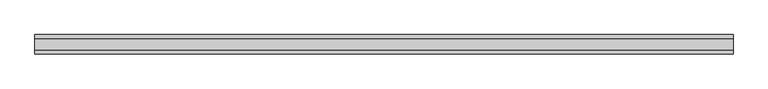
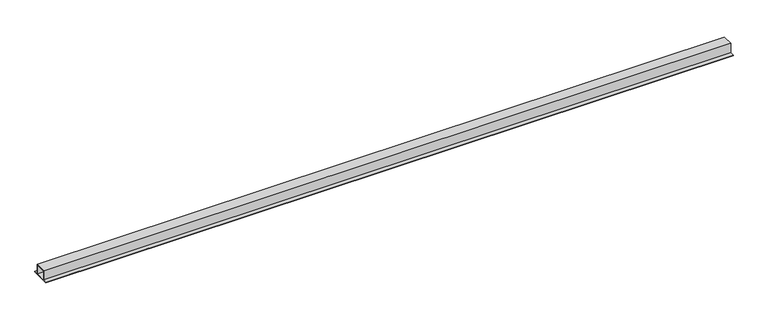
"""IFC4 building model written with IfcOpenShell, lengths in millimetres: beam geometry, NLRS_28_SF_LIB_stalen ligger THQ-AV-CWV-MMBS-SRP_gen_rsf : stalen ligger_gen__THQ_280x10-290x30-550x20."""

import ifcopenshell
import ifcopenshell.guid

model = None  # the IFC model being written
_history = None  # IfcOwnerHistory: only IFC2X3 demands one
_inside = {}  # id of a spatial element -> (the spatial element, [elements in it])
_under = {}  # id of a project, library or spatial element -> (it, [spatial elements below it])
_declared = {}  # id of a project -> (the project, [libraries it declares])
_typed = {}  # id of a type object -> (the type object, [elements of that type])
_made_of = {}  # id of a material, layer set ... -> (it, [elements and type objects made of it])


def new_model(schema):
    """Start an empty IFC model of exactly this schema.

    Asked for "IFC4X3", IfcOpenShell would pick the latest addendum, in which some entities
    have other attributes; the version numbers below select the first issue.
    IFC2X3 requires an IfcOwnerHistory on every rooted entity: one is made here for all.
    """
    global model, _history
    if schema == "IFC4X3":
        model = ifcopenshell.file(schema_version=(4, 3, 0, 0))
    else:
        model = ifcopenshell.file(schema=schema)
    _inside.clear()
    _under.clear()
    _declared.clear()
    _typed.clear()
    _made_of.clear()
    _history = None
    if model.schema == "IFC2X3":
        org = make("IfcOrganization", Name="unknown")
        user = make(
            "IfcPersonAndOrganization",
            ThePerson=make("IfcPerson", FamilyName="unknown"),
            TheOrganization=org,
        )
        app = make(
            "IfcApplication",
            ApplicationDeveloper=org,
            Version="unknown",
            ApplicationFullName="unknown",
            ApplicationIdentifier="unknown",
        )
        _history = make(
            "IfcOwnerHistory",
            OwningUser=user,
            OwningApplication=app,
            ChangeAction="ADDED",
            CreationDate=0,
        )
    return model


def make(cls, **values):
    """One entity of the class cls with the attributes given. An attribute that is None is left unset."""
    return model.create_entity(
        cls, **{name: value for name, value in values.items() if value is not None}
    )


def rooted(cls, **values):
    """An entity with a GlobalId (a new one), such as an element, a storey or a relation."""
    return make(cls, GlobalId=ifcopenshell.guid.new(), OwnerHistory=_history, **values)


def si_unit(unit_type, name, prefix=None):
    """IfcSIUnit, for example si_unit("LENGTHUNIT", "METRE", prefix="MILLI")."""
    return make("IfcSIUnit", UnitType=unit_type, Prefix=prefix, Name=name)


def assignment(units):
    """IfcUnitAssignment: the units of a project."""
    return None if units is None else make("IfcUnitAssignment", Units=units)


def point(xyz):
    """IfcCartesianPoint."""
    return None if xyz is None else make("IfcCartesianPoint", Coordinates=xyz)


def direction(xyz):
    """IfcDirection."""
    return None if xyz is None else make("IfcDirection", DirectionRatios=xyz)


def frame(location, z_axis=None, x_axis=None):
    """IfcAxis2Placement3D, a coordinate frame: its origin and axes. An axis left out is left unset."""
    return make(
        "IfcAxis2Placement3D",
        Location=point(location),
        Axis=direction(z_axis),
        RefDirection=direction(x_axis),
    )


def origin():
    """The frame at (0, 0, 0) with its axes left unset."""
    return frame((0.0, 0.0, 0.0))


def place(relative_to, where):
    """IfcLocalPlacement: puts the frame where relative to a parent placement (None: the world)."""
    return make(
        "IfcLocalPlacement", PlacementRelTo=relative_to, RelativePlacement=where
    )


def context(
    kind, dimensions, precision=None, world=None, true_north=None, identifier=None
):
    """IfcGeometricRepresentationContext, for example the 3D "Model" context."""
    return make(
        "IfcGeometricRepresentationContext",
        ContextIdentifier=identifier,
        ContextType=kind,
        CoordinateSpaceDimension=dimensions,
        Precision=precision,
        WorldCoordinateSystem=world,
        TrueNorth=true_north,
    )


def project(units=None, contexts=None):
    """IfcProject with its units and contexts."""
    return rooted(
        "IfcProject",
        Name="project",
        RepresentationContexts=contexts,
        UnitsInContext=assignment(units),
    )


def spatial(cls, under=None, at=None, **own):
    """A site, building, storey or space (cls), placed at a placement, below another one or the project."""
    s = rooted(cls, ObjectPlacement=at, **own)
    if under is not None:
        _under.setdefault(under.id(), (under, []))[1].append(s)
    return s


def polyline(points):
    """IfcPolyline through the points."""
    return make("IfcPolyline", Points=[point(p) for p in points])


def outline(outer, holes=None, kind="AREA"):
    """IfcArbitraryClosedProfileDef: a profile drawn as a closed curve; with holes, ...WithVoids."""
    if holes is None:
        return make("IfcArbitraryClosedProfileDef", ProfileType=kind, OuterCurve=outer)
    return make(
        "IfcArbitraryProfileDefWithVoids",
        ProfileType=kind,
        OuterCurve=outer,
        InnerCurves=holes,
    )


def extrude(swept, where, along, depth):
    """IfcExtrudedAreaSolid: the profile swept, set in the frame where, extruded along a direction by depth."""
    return make(
        "IfcExtrudedAreaSolid",
        SweptArea=swept,
        Position=where,
        ExtrudedDirection=direction(along),
        Depth=depth,
    )


def shape(context_of_items, identifier, shape_type, items):
    """IfcShapeRepresentation: the items that make up one representation, for example the "Body"."""
    return make(
        "IfcShapeRepresentation",
        ContextOfItems=context_of_items,
        RepresentationIdentifier=identifier,
        RepresentationType=shape_type,
        Items=items,
    )


def source(mapping_origin, context_of_items, identifier, shape_type, items):
    """IfcRepresentationMap: a shape defined once, which mapped items show again and again."""
    return make(
        "IfcRepresentationMap",
        MappingOrigin=mapping_origin,
        MappedRepresentation=shape(context_of_items, identifier, shape_type, items),
    )


def transform(
    local_origin,
    x_axis=None,
    y_axis=None,
    z_axis=None,
    scale=None,
    scale2=None,
    scale3=None,
    uniform=True,
):
    """IfcCartesianTransformationOperator3D, or its non-uniform kind. x_axis, y_axis, z_axis: its Axis1, 2, 3."""
    if uniform:
        return make(
            "IfcCartesianTransformationOperator3D",
            Axis1=direction(x_axis),
            Axis2=direction(y_axis),
            LocalOrigin=point(local_origin),
            Scale=scale,
            Axis3=direction(z_axis),
        )
    return make(
        "IfcCartesianTransformationOperator3DnonUniform",
        Axis1=direction(x_axis),
        Axis2=direction(y_axis),
        LocalOrigin=point(local_origin),
        Scale=scale,
        Axis3=direction(z_axis),
        Scale2=scale2,
        Scale3=scale3,
    )


def mapped(mapping_source, mapping_target):
    """IfcMappedItem: shows the shape of a source again, moved by a transform."""
    return make(
        "IfcMappedItem", MappingSource=mapping_source, MappingTarget=mapping_target
    )


def made_of(thing, what):
    """Note that an element or type object is made of a material, layer set ...; save() writes the relation."""
    if what is not None:
        _made_of.setdefault(what.id(), (what, []))[1].append(thing)
    return thing


def element(
    cls,
    number,
    at=None,
    inside=None,
    cuts=None,
    type_object=None,
    material=None,
    context=None,
    identifier="Body",
    shape_type=None,
    held_by="IfcProductDefinitionShape",
    body=None,
    shapes=None,
    **own,
):
    """One element of the class cls, such as IfcWall. Its Tag is "e" and its number.

    at: its placement. inside: the storey or other place that contains it. cuts: it is an
    opening in that element (IfcRelVoidsElement). A single representation is given by context,
    identifier, shape_type and body (its items); several are given by shapes. held_by: the class
    of the entity that holds the representations. save() writes the other relations.
    """
    e = rooted(cls, Tag="e%d" % number, ObjectPlacement=at, **own)
    if body is not None:
        shapes = [shape(context, identifier, shape_type, body)]
    if shapes is not None:
        e.Representation = make(held_by, Representations=shapes)
    if inside is not None:
        _inside.setdefault(inside.id(), (inside, []))[1].append(e)
    if cuts is not None:
        rooted(
            "IfcRelVoidsElement", RelatingBuildingElement=cuts, RelatedOpeningElement=e
        )
    if type_object is not None:
        _typed.setdefault(type_object.id(), (type_object, []))[1].append(e)
    return made_of(e, material)


def aggregate(whole, parts):
    """IfcRelAggregates: a whole, such as a stair, and the parts it consists of."""
    return rooted("IfcRelAggregates", RelatingObject=whole, RelatedObjects=parts)


def save(model, path):
    """Write the relations noted so far, then the file.

    IfcRelAggregates (storeys below a building ...), IfcRelContainedInSpatialStructure (elements
    in a storey), IfcRelDefinesByType, IfcRelAssociatesMaterial and IfcRelDeclares: one each for
    every whole, place, type object, material and project.
    """
    for whole, parts in _under.values():
        aggregate(whole, parts)
    for where, things in _inside.values():
        rooted(
            "IfcRelContainedInSpatialStructure",
            RelatedElements=things,
            RelatingStructure=where,
        )
    for kind, things in _typed.values():
        rooted("IfcRelDefinesByType", RelatedObjects=things, RelatingType=kind)
    for what, things in _made_of.values():
        rooted("IfcRelAssociatesMaterial", RelatedObjects=things, RelatingMaterial=what)
    for by, libraries in _declared.values():
        rooted("IfcRelDeclares", RelatingContext=by, RelatedDefinitions=libraries)
    model.write(path)


def beam_1759c74d(model_context):
    return source(origin(), model_context, "Body", "SweptSolid", [
        extrude(outline(polyline([(143.5, 280.0), (143.5, 0.0), (263.5, 0.0), (263.5, -20.0), (-286.5, -20.0), (-286.5, 0.0), (-166.5, 0.0), (-166.5, 280.0), (143.5, 280.0)]), holes=[polyline([(133.5, 0.0), (133.5, 250.0), (-156.5, 250.0), (-156.5, 0.0), (133.5, 0.0)])]), frame((-9887.5, 0.0, 0.0), z_axis=(1.0, 0.0, 0.0), x_axis=(0.0, 1.0, 0.0)), (0.0, 0.0, 1.0), 19775.0),
    ])


if __name__ == "__main__":
    model = new_model("IFC4")
    model_context = context("Model", 3, world=origin())
    ifc_project = project(units=[si_unit("LENGTHUNIT", "METRE", prefix="MILLI")], contexts=[model_context])
    site = spatial("IfcSite", under=ifc_project)
    building = spatial("IfcBuilding", under=site)
    placement = place(None, origin())
    beam_shape = beam_1759c74d(model_context)
    element("IfcBeam", 1, ObjectType="NLRS_28_SF_LIB_stalen ligger THQ-AV-CWV-MMBS-SRP_gen_rsf : stalen ligger_gen__THQ_280x10-290x30-550x20", at=placement, inside=building, context=model_context, shape_type="MappedRepresentation", body=[
        mapped(beam_shape, transform((0.0, 0.0, 0.0), x_axis=(1.0, 0.0, 0.0), y_axis=(0.0, 1.0, 0.0), z_axis=(0.0, 0.0, 1.0))),
    ])
    save(model, "model.ifc")

# Revit data of these elements
# Type "NLRS_28_SF_LIB_stalen ligger THQ-AV-CWV-MMBS-SRP_gen_rsf : stalen ligger_gen__THQ_280x10-290x30-550x20"
#   Export Type to IFC As = "IfcBeamType"
#   Type IfcGUID = "2GRbcre991teoKeCLB8MAm"
#   Type Comments = "THQ 280x10-290x30-550x20"
#   Model = " "
#   Manufacturer = " "
#   Fire Rating = " "
#   Description = "stalen ligger THQ 280x10-290x30-550x20"
#   Assembly Code = "28.11"
#   tw = 10 mm
#   tu = 20 mm
#   to = 30 mm
#   h = 280 mm
#   bu = 550 mm
#   bo = 290 mm
#   NLRS_C_lengte [instance default] = 1500 mm
#   Length [instance default] = 1500 mm
#   RSF_C_vullen_met_beton [instance default] = no
#   RSF_C_petligger = no
#   RSF_C_hoedligger = yes
#   Structural Material = NLRS_h2_staal_gen_rsf
#   Keynote = ""
# Element 1 (IfcBeam, "NLRS_28_SF_LIB_stalen ligger THQ-AV-CWV-MMBS-SRP_gen_rsf : stalen ligger_gen__THQ_280x10-290x30-550x20")
#   NLRS_C_lengte = 19775 mm
#   Materials on its faces: "NLRS_h2_staal_gen_rsf"
# Materials
#   "NLRS_h2_staal_gen_rsf": class "H - Metaal", colour RGB 189 187 185, transparency 0, Keynote = "h2", Manufacturer = "Revit Standards Foundation", URL = "www.revitstandards.org", Description = "staal", Cost = 0
